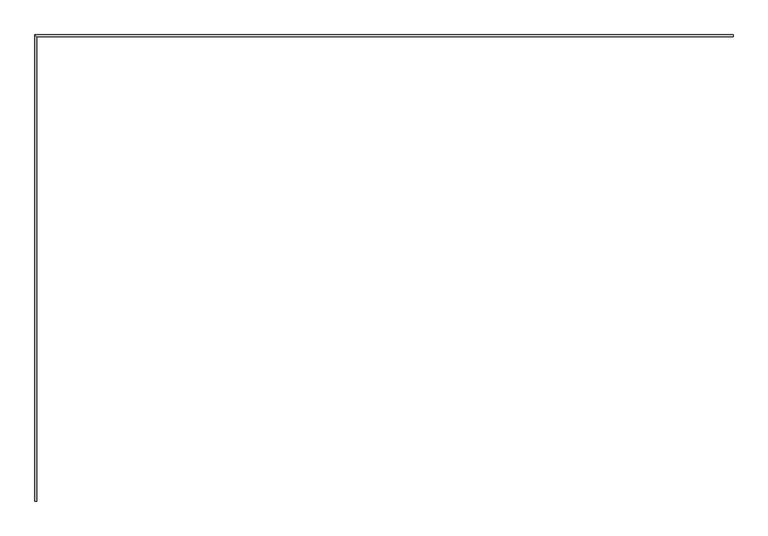
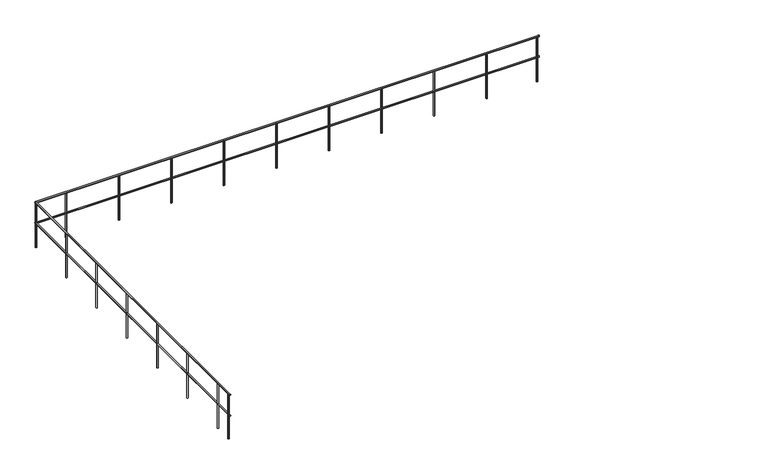
"""IFC4 building model written with IfcOpenShell, lengths in millimetres: railing geometry."""

from ifc_helpers import new_model, si_unit, point, frame, frame_2d, origin, place, context, project, spatial, circle_curve, ellipse_curve, trimmed, segment, composite_curve, outline, extrude, source, transform, mapped, element, save
from ifc_brep_helpers import plane_surface, cylinder_surface, advanced_brep


def railing_3e9f266b(model_context):
    return source(origin(), model_context, "Body", "SolidModel", [
        advanced_brep(
        [(3975.7243044, 65167.0208589, 885.0), (3975.7243044, 65137.0208589, 885.0), (-7501.0, 65137.0208589, 885.0), (-7531.0, 65167.0208589, 885.0), (-7531.0, 57477.0208589, 885.0), (-7501.0, 57477.0208589, 885.0)],
        [
            (0, 1, circle_curve(frame((3975.7243044, 65152.0208589, 885.0), z_axis=(1.0, 0.0, 0.0), x_axis=(0.0, -1.0, 0.0)), 15.0)),
            (1, 0, circle_curve(frame((3975.7243044, 65152.0208589, 885.0), z_axis=(1.0, 0.0, 0.0), x_axis=(0.0, -1.0, 0.0)), 15.0)),
            (1, 2),
            (2, 3, ellipse_curve(frame((-7516.0, 65152.0208589, 885.0), z_axis=(0.7071067811865491, 0.7071067811865459, 0.0), x_axis=(0.7071067811865458, -0.7071067811865491, 0.0)), 21.2132034, 15.0)),
            (3, 0),
            (3, 2, ellipse_curve(frame((-7516.0, 65152.0208589, 885.0), z_axis=(0.7071067811865491, 0.7071067811865459, 0.0), x_axis=(0.7071067811865458, -0.7071067811865491, 0.0)), 21.2132034, 15.0)),
            (4, 5, circle_curve(frame((-7516.0, 57477.0208589, 885.0), z_axis=(0.0, -1.0, 0.0), x_axis=(1.0, 0.0, 0.0)), 15.0)),
            (5, 4, circle_curve(frame((-7516.0, 57477.0208589, 885.0), z_axis=(0.0, -1.0, 0.0), x_axis=(1.0, 0.0, 0.0)), 15.0)),
            (2, 5),
            (4, 3),
        ],
        [
            plane_surface(frame((3975.7243044, 65152.0208589, 900.0), z_axis=(1.0, 0.0, 0.0), x_axis=(0.0, -1.0, 0.0))),
            cylinder_surface(frame((3975.7243044, 65152.0208589, 885.0), z_axis=(1.0, 0.0, 0.0), x_axis=(0.0, -1.0, 0.0)), 15.0),
            plane_surface(frame((-7516.0, 57477.0208589, 900.0), z_axis=(0.0, -1.0, 0.0), x_axis=(0.0, 0.0, -1.0))),
            cylinder_surface(frame((-7516.0, 65152.0208589, 885.0), z_axis=(0.0, 1.0, 0.0), x_axis=(1.0, 0.0, 0.0)), 15.0),
        ],
        [
            (0, [[1, 2]]),
            (1, [[-2, 3, 4, 5]]),
            (1, [[-1, -5, 6, -3]]),
            (2, [[7, 8]]),
            (3, [[-4, 9, -7, 10]]),
            (3, [[-6, -10, -8, -9]]),
        ],
    ),
        advanced_brep(
        [(3975.7243044, 65167.0208589, 1385.0), (3975.7243044, 65137.0208589, 1385.0), (-7501.0, 65137.0208589, 1385.0), (-7531.0, 65167.0208589, 1385.0), (-7531.0, 57477.0208589, 1385.0), (-7501.0, 57477.0208589, 1385.0)],
        [
            (0, 1, circle_curve(frame((3975.7243044, 65152.0208589, 1385.0), z_axis=(1.0, 0.0, 0.0), x_axis=(0.0, -1.0, 0.0)), 15.0)),
            (1, 0, circle_curve(frame((3975.7243044, 65152.0208589, 1385.0), z_axis=(1.0, 0.0, 0.0), x_axis=(0.0, -1.0, 0.0)), 15.0)),
            (1, 2),
            (2, 3, ellipse_curve(frame((-7516.0, 65152.0208589, 1385.0), z_axis=(0.7071067811865491, 0.7071067811865459, 0.0), x_axis=(0.7071067811865458, -0.7071067811865491, 0.0)), 21.2132034, 15.0)),
            (3, 0),
            (3, 2, ellipse_curve(frame((-7516.0, 65152.0208589, 1385.0), z_axis=(0.7071067811865491, 0.7071067811865459, 0.0), x_axis=(0.7071067811865458, -0.7071067811865491, 0.0)), 21.2132034, 15.0)),
            (4, 5, circle_curve(frame((-7516.0, 57477.0208589, 1385.0), z_axis=(0.0, -1.0, 0.0), x_axis=(1.0, 0.0, 0.0)), 15.0)),
            (5, 4, circle_curve(frame((-7516.0, 57477.0208589, 1385.0), z_axis=(0.0, -1.0, 0.0), x_axis=(1.0, 0.0, 0.0)), 15.0)),
            (2, 5),
            (4, 3),
        ],
        [
            plane_surface(frame((3975.7243044, 65152.0208589, 1400.0), z_axis=(1.0, 0.0, 0.0), x_axis=(0.0, -1.0, 0.0))),
            cylinder_surface(frame((3975.7243044, 65152.0208589, 1385.0), z_axis=(1.0, 0.0, 0.0), x_axis=(0.0, -1.0, 0.0)), 15.0),
            plane_surface(frame((-7516.0, 57477.0208589, 1400.0), z_axis=(0.0, -1.0, 0.0), x_axis=(0.0, 0.0, -1.0))),
            cylinder_surface(frame((-7516.0, 65152.0208589, 1385.0), z_axis=(0.0, 1.0, 0.0), x_axis=(1.0, 0.0, 0.0)), 15.0),
        ],
        [
            (0, [[1, 2]]),
            (1, [[-2, 3, 4, 5]]),
            (1, [[-1, -5, 6, -3]]),
            (2, [[7, 8]]),
            (3, [[-4, 9, -7, 10]]),
            (3, [[-6, -10, -8, -9]]),
        ],
    ),
        extrude(outline(composite_curve([segment(trimmed(circle_curve(frame_2d((-7516.0, 57952.0208589)), 15.0), [point((-7531.0, 57952.0208589))], [point((-7501.0, 57952.0208589))], False, "CARTESIAN"), True, "CONTINUOUS"), segment(trimmed(circle_curve(frame_2d((-7516.0, 57952.0208589)), 15.0), [point((-7501.0, 57952.0208589))], [point((-7531.0, 57952.0208589))], False, "CARTESIAN"), True, "CONTINUOUS")], self_intersect=False)), frame((0.0, 0.0, 300.0), z_axis=(0.0, 0.0, 1.0), x_axis=(1.0, 0.0, 0.0)), (0.0, 0.0, 1.0), 1070.0),
        extrude(outline(composite_curve([segment(trimmed(circle_curve(frame_2d((-7516.0, 59152.0208589)), 15.0), [point((-7531.0, 59152.0208589))], [point((-7501.0, 59152.0208589))], False, "CARTESIAN"), True, "CONTINUOUS"), segment(trimmed(circle_curve(frame_2d((-7516.0, 59152.0208589)), 15.0), [point((-7501.0, 59152.0208589))], [point((-7531.0, 59152.0208589))], False, "CARTESIAN"), True, "CONTINUOUS")], self_intersect=False)), frame((0.0, 0.0, 300.0), z_axis=(0.0, 0.0, 1.0), x_axis=(1.0, 0.0, 0.0)), (0.0, 0.0, 1.0), 1070.0),
        extrude(outline(composite_curve([segment(trimmed(circle_curve(frame_2d((-7516.0, 60352.0208589)), 15.0), [point((-7531.0, 60352.0208589))], [point((-7501.0, 60352.0208589))], False, "CARTESIAN"), True, "CONTINUOUS"), segment(trimmed(circle_curve(frame_2d((-7516.0, 60352.0208589)), 15.0), [point((-7501.0, 60352.0208589))], [point((-7531.0, 60352.0208589))], False, "CARTESIAN"), True, "CONTINUOUS")], self_intersect=False)), frame((0.0, 0.0, 300.0), z_axis=(0.0, 0.0, 1.0), x_axis=(1.0, 0.0, 0.0)), (0.0, 0.0, 1.0), 1070.0),
        extrude(outline(composite_curve([segment(trimmed(circle_curve(frame_2d((-7516.0, 61552.0208589)), 15.0), [point((-7531.0, 61552.0208589))], [point((-7501.0, 61552.0208589))], False, "CARTESIAN"), True, "CONTINUOUS"), segment(trimmed(circle_curve(frame_2d((-7516.0, 61552.0208589)), 15.0), [point((-7501.0, 61552.0208589))], [point((-7531.0, 61552.0208589))], False, "CARTESIAN"), True, "CONTINUOUS")], self_intersect=False)), frame((0.0, 0.0, 300.0), z_axis=(0.0, 0.0, 1.0), x_axis=(1.0, 0.0, 0.0)), (0.0, 0.0, 1.0), 1070.0),
        extrude(outline(composite_curve([segment(trimmed(circle_curve(frame_2d((-7516.0, 62752.0208589)), 15.0), [point((-7531.0, 62752.0208589))], [point((-7501.0, 62752.0208589))], False, "CARTESIAN"), True, "CONTINUOUS"), segment(trimmed(circle_curve(frame_2d((-7516.0, 62752.0208589)), 15.0), [point((-7501.0, 62752.0208589))], [point((-7531.0, 62752.0208589))], False, "CARTESIAN"), True, "CONTINUOUS")], self_intersect=False)), frame((0.0, 0.0, 300.0), z_axis=(0.0, 0.0, 1.0), x_axis=(1.0, 0.0, 0.0)), (0.0, 0.0, 1.0), 1070.0),
        extrude(outline(composite_curve([segment(trimmed(circle_curve(frame_2d((-7516.0, 63952.0208589)), 15.0), [point((-7531.0, 63952.0208589))], [point((-7501.0, 63952.0208589))], False, "CARTESIAN"), True, "CONTINUOUS"), segment(trimmed(circle_curve(frame_2d((-7516.0, 63952.0208589)), 15.0), [point((-7501.0, 63952.0208589))], [point((-7531.0, 63952.0208589))], False, "CARTESIAN"), True, "CONTINUOUS")], self_intersect=False)), frame((0.0, 0.0, 300.0), z_axis=(0.0, 0.0, 1.0), x_axis=(1.0, 0.0, 0.0)), (0.0, 0.0, 1.0), 1070.0),
        extrude(outline(composite_curve([segment(trimmed(circle_curve(frame_2d((-6824.2756956, 65152.0208589)), 15.0), [point((-6824.2756956, 65167.0208589))], [point((-6824.2756956, 65137.0208589))], False, "CARTESIAN"), True, "CONTINUOUS"), segment(trimmed(circle_curve(frame_2d((-6824.2756956, 65152.0208589)), 15.0), [point((-6824.2756956, 65137.0208589))], [point((-6824.2756956, 65167.0208589))], False, "CARTESIAN"), True, "CONTINUOUS")], self_intersect=False)), frame((0.0, 0.0, 300.0), z_axis=(0.0, 0.0, 1.0), x_axis=(1.0, 0.0, 0.0)), (0.0, 0.0, 1.0), 1070.0),
        extrude(outline(composite_curve([segment(trimmed(circle_curve(frame_2d((-5624.2756956, 65152.0208589)), 15.0), [point((-5624.2756956, 65167.0208589))], [point((-5624.2756956, 65137.0208589))], False, "CARTESIAN"), True, "CONTINUOUS"), segment(trimmed(circle_curve(frame_2d((-5624.2756956, 65152.0208589)), 15.0), [point((-5624.2756956, 65137.0208589))], [point((-5624.2756956, 65167.0208589))], False, "CARTESIAN"), True, "CONTINUOUS")], self_intersect=False)), frame((0.0, 0.0, 300.0), z_axis=(0.0, 0.0, 1.0), x_axis=(1.0, 0.0, 0.0)), (0.0, 0.0, 1.0), 1070.0),
        extrude(outline(composite_curve([segment(trimmed(circle_curve(frame_2d((-4424.2756956, 65152.0208589)), 15.0), [point((-4424.2756956, 65167.0208589))], [point((-4424.2756956, 65137.0208589))], False, "CARTESIAN"), True, "CONTINUOUS"), segment(trimmed(circle_curve(frame_2d((-4424.2756956, 65152.0208589)), 15.0), [point((-4424.2756956, 65137.0208589))], [point((-4424.2756956, 65167.0208589))], False, "CARTESIAN"), True, "CONTINUOUS")], self_intersect=False)), frame((0.0, 0.0, 300.0), z_axis=(0.0, 0.0, 1.0), x_axis=(1.0, 0.0, 0.0)), (0.0, 0.0, 1.0), 1070.0),
        extrude(outline(composite_curve([segment(trimmed(circle_curve(frame_2d((-3224.2756956, 65152.0208589)), 15.0), [point((-3224.2756956, 65167.0208589))], [point((-3224.2756956, 65137.0208589))], False, "CARTESIAN"), True, "CONTINUOUS"), segment(trimmed(circle_curve(frame_2d((-3224.2756956, 65152.0208589)), 15.0), [point((-3224.2756956, 65137.0208589))], [point((-3224.2756956, 65167.0208589))], False, "CARTESIAN"), True, "CONTINUOUS")], self_intersect=False)), frame((0.0, 0.0, 300.0), z_axis=(0.0, 0.0, 1.0), x_axis=(1.0, 0.0, 0.0)), (0.0, 0.0, 1.0), 1070.0),
        extrude(outline(composite_curve([segment(trimmed(circle_curve(frame_2d((-2024.2756956, 65152.0208589)), 15.0), [point((-2024.2756956, 65167.0208589))], [point((-2024.2756956, 65137.0208589))], False, "CARTESIAN"), True, "CONTINUOUS"), segment(trimmed(circle_curve(frame_2d((-2024.2756956, 65152.0208589)), 15.0), [point((-2024.2756956, 65137.0208589))], [point((-2024.2756956, 65167.0208589))], False, "CARTESIAN"), True, "CONTINUOUS")], self_intersect=False)), frame((0.0, 0.0, 300.0), z_axis=(0.0, 0.0, 1.0), x_axis=(1.0, 0.0, 0.0)), (0.0, 0.0, 1.0), 1070.0),
        extrude(outline(composite_curve([segment(trimmed(circle_curve(frame_2d((-824.2756956, 65152.0208589)), 15.0), [point((-824.2756956, 65167.0208589))], [point((-824.2756956, 65137.0208589))], False, "CARTESIAN"), True, "CONTINUOUS"), segment(trimmed(circle_curve(frame_2d((-824.2756956, 65152.0208589)), 15.0), [point((-824.2756956, 65137.0208589))], [point((-824.2756956, 65167.0208589))], False, "CARTESIAN"), True, "CONTINUOUS")], self_intersect=False)), frame((0.0, 0.0, 300.0), z_axis=(0.0, 0.0, 1.0), x_axis=(1.0, 0.0, 0.0)), (0.0, 0.0, 1.0), 1070.0),
        extrude(outline(composite_curve([segment(trimmed(circle_curve(frame_2d((375.7243044, 65152.0208589)), 15.0), [point((375.7243044, 65167.0208589))], [point((375.7243044, 65137.0208589))], False, "CARTESIAN"), True, "CONTINUOUS"), segment(trimmed(circle_curve(frame_2d((375.7243044, 65152.0208589)), 15.0), [point((375.7243044, 65137.0208589))], [point((375.7243044, 65167.0208589))], False, "CARTESIAN"), True, "CONTINUOUS")], self_intersect=False)), frame((0.0, 0.0, 300.0), z_axis=(0.0, 0.0, 1.0), x_axis=(1.0, 0.0, 0.0)), (0.0, 0.0, 1.0), 1070.0),
        extrude(outline(composite_curve([segment(trimmed(circle_curve(frame_2d((1575.7243044, 65152.0208589)), 15.0), [point((1575.7243044, 65167.0208589))], [point((1575.7243044, 65137.0208589))], False, "CARTESIAN"), True, "CONTINUOUS"), segment(trimmed(circle_curve(frame_2d((1575.7243044, 65152.0208589)), 15.0), [point((1575.7243044, 65137.0208589))], [point((1575.7243044, 65167.0208589))], False, "CARTESIAN"), True, "CONTINUOUS")], self_intersect=False)), frame((0.0, 0.0, 300.0), z_axis=(0.0, 0.0, 1.0), x_axis=(1.0, 0.0, 0.0)), (0.0, 0.0, 1.0), 1070.0),
        extrude(outline(composite_curve([segment(trimmed(circle_curve(frame_2d((2775.7243044, 65152.0208589)), 15.0), [point((2775.7243044, 65167.0208589))], [point((2775.7243044, 65137.0208589))], False, "CARTESIAN"), True, "CONTINUOUS"), segment(trimmed(circle_curve(frame_2d((2775.7243044, 65152.0208589)), 15.0), [point((2775.7243044, 65137.0208589))], [point((2775.7243044, 65167.0208589))], False, "CARTESIAN"), True, "CONTINUOUS")], self_intersect=False)), frame((0.0, 0.0, 300.0), z_axis=(0.0, 0.0, 1.0), x_axis=(1.0, 0.0, 0.0)), (0.0, 0.0, 1.0), 1070.0),
        extrude(outline(composite_curve([segment(trimmed(circle_curve(frame_2d((-7516.0, 65152.0208589)), 15.0), [point((-7516.0, 65167.0208589))], [point((-7516.0, 65137.0208589))], False, "CARTESIAN"), True, "CONTINUOUS"), segment(trimmed(circle_curve(frame_2d((-7516.0, 65152.0208589)), 15.0), [point((-7516.0, 65137.0208589))], [point((-7516.0, 65167.0208589))], False, "CARTESIAN"), True, "CONTINUOUS")], self_intersect=False)), frame((0.0, 0.0, 300.0), z_axis=(0.0, 0.0, 1.0), x_axis=(1.0, 0.0, 0.0)), (0.0, 0.0, 1.0), 1070.0),
        extrude(outline(composite_curve([segment(trimmed(circle_curve(frame_2d((-7516.0, 57527.0208589)), 15.0), [point((-7531.0, 57527.0208589))], [point((-7501.0, 57527.0208589))], False, "CARTESIAN"), True, "CONTINUOUS"), segment(trimmed(circle_curve(frame_2d((-7516.0, 57527.0208589)), 15.0), [point((-7501.0, 57527.0208589))], [point((-7531.0, 57527.0208589))], False, "CARTESIAN"), True, "CONTINUOUS")], self_intersect=False)), frame((0.0, 0.0, 300.0), z_axis=(0.0, 0.0, 1.0), x_axis=(1.0, 0.0, 0.0)), (0.0, 0.0, 1.0), 1070.0),
        extrude(outline(composite_curve([segment(trimmed(circle_curve(frame_2d((3925.7243044, 65152.0208589)), 15.0), [point((3925.7243044, 65167.0208589))], [point((3925.7243044, 65137.0208589))], False, "CARTESIAN"), True, "CONTINUOUS"), segment(trimmed(circle_curve(frame_2d((3925.7243044, 65152.0208589)), 15.0), [point((3925.7243044, 65137.0208589))], [point((3925.7243044, 65167.0208589))], False, "CARTESIAN"), True, "CONTINUOUS")], self_intersect=False)), frame((0.0, 0.0, 300.0), z_axis=(0.0, 0.0, 1.0), x_axis=(1.0, 0.0, 0.0)), (0.0, 0.0, 1.0), 1070.0),
    ])


if __name__ == "__main__":
    model = new_model("IFC4")
    model_context = context("Model", 3, world=origin())
    ifc_project = project(units=[si_unit("LENGTHUNIT", "METRE", prefix="MILLI")], contexts=[model_context])
    site = spatial("IfcSite", under=ifc_project)
    building = spatial("IfcBuilding", under=site)
    placement = place(None, origin())
    railing_shape = railing_3e9f266b(model_context)
    element("IfcRailing", 1, at=placement, inside=building, context=model_context, shape_type="MappedRepresentation", body=[
        mapped(railing_shape, transform((0.0, 0.0, 0.0), x_axis=(1.0, 0.0, 0.0), y_axis=(0.0, 1.0, 0.0), z_axis=(0.0, 0.0, 1.0))),
    ])
    save(model, "model.ifc")
